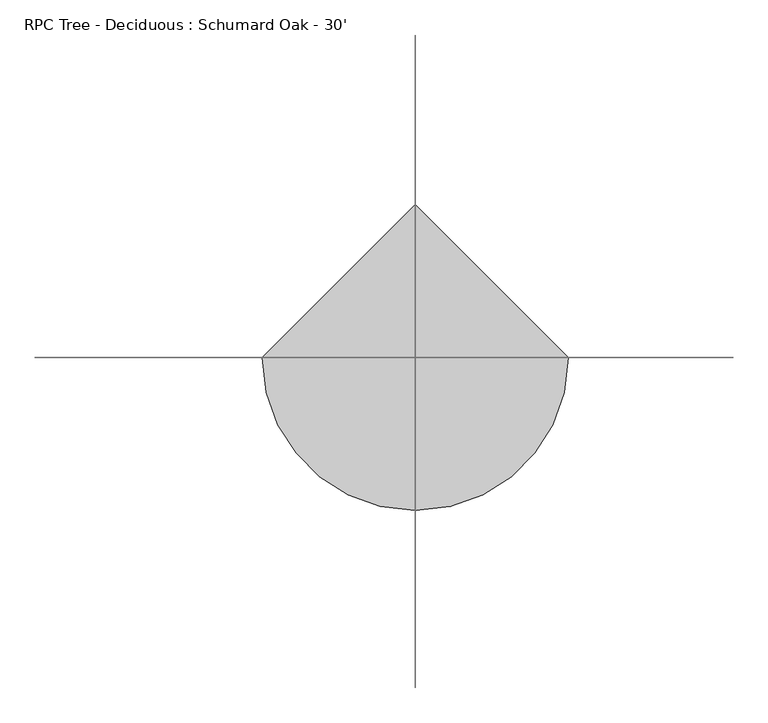
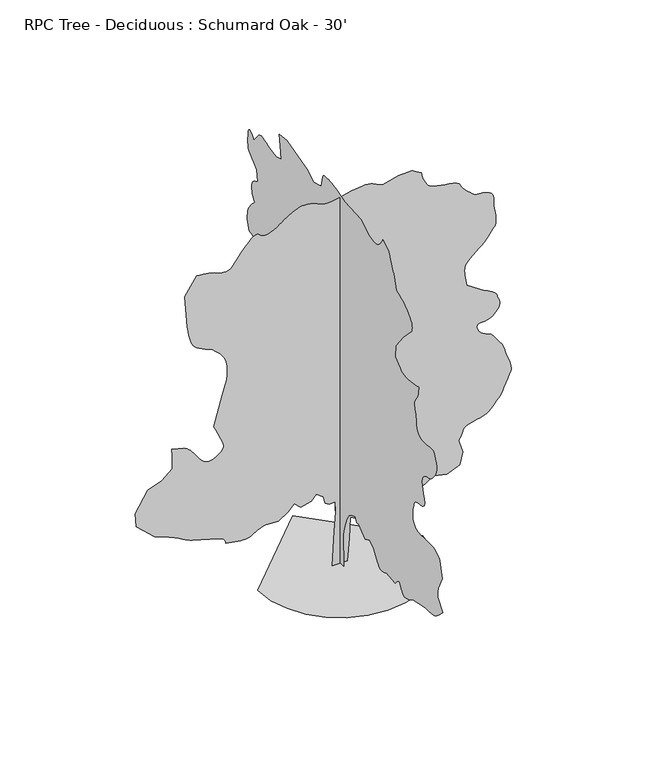
"""IFC4 building model written with IfcOpenShell, lengths in millimetres: geographic element geometry, RPC Tree - Deciduous : Schumard Oak - 30'."""

import ifcopenshell
import ifcopenshell.guid

model = None  # the IFC model being written
_history = None  # IfcOwnerHistory: only IFC2X3 demands one
_inside = {}  # id of a spatial element -> (the spatial element, [elements in it])
_under = {}  # id of a project, library or spatial element -> (it, [spatial elements below it])
_declared = {}  # id of a project -> (the project, [libraries it declares])
_typed = {}  # id of a type object -> (the type object, [elements of that type])
_made_of = {}  # id of a material, layer set ... -> (it, [elements and type objects made of it])


def new_model(schema):
    """Start an empty IFC model of exactly this schema.

    Asked for "IFC4X3", IfcOpenShell would pick the latest addendum, in which some entities
    have other attributes; the version numbers below select the first issue.
    IFC2X3 requires an IfcOwnerHistory on every rooted entity: one is made here for all.
    """
    global model, _history
    if schema == "IFC4X3":
        model = ifcopenshell.file(schema_version=(4, 3, 0, 0))
    else:
        model = ifcopenshell.file(schema=schema)
    _inside.clear()
    _under.clear()
    _declared.clear()
    _typed.clear()
    _made_of.clear()
    _history = None
    if model.schema == "IFC2X3":
        org = make("IfcOrganization", Name="unknown")
        user = make(
            "IfcPersonAndOrganization",
            ThePerson=make("IfcPerson", FamilyName="unknown"),
            TheOrganization=org,
        )
        app = make(
            "IfcApplication",
            ApplicationDeveloper=org,
            Version="unknown",
            ApplicationFullName="unknown",
            ApplicationIdentifier="unknown",
        )
        _history = make(
            "IfcOwnerHistory",
            OwningUser=user,
            OwningApplication=app,
            ChangeAction="ADDED",
            CreationDate=0,
        )
    return model


def make(cls, **values):
    """One entity of the class cls with the attributes given. An attribute that is None is left unset."""
    return model.create_entity(
        cls, **{name: value for name, value in values.items() if value is not None}
    )


def rooted(cls, **values):
    """An entity with a GlobalId (a new one), such as an element, a storey or a relation."""
    return make(cls, GlobalId=ifcopenshell.guid.new(), OwnerHistory=_history, **values)


def si_unit(unit_type, name, prefix=None):
    """IfcSIUnit, for example si_unit("LENGTHUNIT", "METRE", prefix="MILLI")."""
    return make("IfcSIUnit", UnitType=unit_type, Prefix=prefix, Name=name)


def assignment(units):
    """IfcUnitAssignment: the units of a project."""
    return None if units is None else make("IfcUnitAssignment", Units=units)


def point(xyz):
    """IfcCartesianPoint."""
    return None if xyz is None else make("IfcCartesianPoint", Coordinates=xyz)


def direction(xyz):
    """IfcDirection."""
    return None if xyz is None else make("IfcDirection", DirectionRatios=xyz)


def frame(location, z_axis=None, x_axis=None):
    """IfcAxis2Placement3D, a coordinate frame: its origin and axes. An axis left out is left unset."""
    return make(
        "IfcAxis2Placement3D",
        Location=point(location),
        Axis=direction(z_axis),
        RefDirection=direction(x_axis),
    )


def origin():
    """The frame at (0, 0, 0) with its axes left unset."""
    return frame((0.0, 0.0, 0.0))


def place(relative_to, where):
    """IfcLocalPlacement: puts the frame where relative to a parent placement (None: the world)."""
    return make(
        "IfcLocalPlacement", PlacementRelTo=relative_to, RelativePlacement=where
    )


def context(
    kind, dimensions, precision=None, world=None, true_north=None, identifier=None
):
    """IfcGeometricRepresentationContext, for example the 3D "Model" context."""
    return make(
        "IfcGeometricRepresentationContext",
        ContextIdentifier=identifier,
        ContextType=kind,
        CoordinateSpaceDimension=dimensions,
        Precision=precision,
        WorldCoordinateSystem=world,
        TrueNorth=true_north,
    )


def project(units=None, contexts=None):
    """IfcProject with its units and contexts."""
    return rooted(
        "IfcProject",
        Name="project",
        RepresentationContexts=contexts,
        UnitsInContext=assignment(units),
    )


def spatial(cls, under=None, at=None, **own):
    """A site, building, storey or space (cls), placed at a placement, below another one or the project."""
    s = rooted(cls, ObjectPlacement=at, **own)
    if under is not None:
        _under.setdefault(under.id(), (under, []))[1].append(s)
    return s


def point_list(points):
    """IfcCartesianPointList2D or 3D."""
    cls = (
        "IfcCartesianPointList2D" if len(points[0]) == 2 else "IfcCartesianPointList3D"
    )
    return make(cls, CoordList=points)


def triangles(points, corners, closed=None, point_numbers=None):
    """IfcTriangulatedFaceSet: each triangle names its three corners, points numbered from 1."""
    return make(
        "IfcTriangulatedFaceSet",
        Coordinates=point_list(points),
        Closed=closed,
        CoordIndex=corners,
        PnIndex=point_numbers,
    )


def shape(context_of_items, identifier, shape_type, items):
    """IfcShapeRepresentation: the items that make up one representation, for example the "Body"."""
    return make(
        "IfcShapeRepresentation",
        ContextOfItems=context_of_items,
        RepresentationIdentifier=identifier,
        RepresentationType=shape_type,
        Items=items,
    )


def source(mapping_origin, context_of_items, identifier, shape_type, items):
    """IfcRepresentationMap: a shape defined once, which mapped items show again and again."""
    return make(
        "IfcRepresentationMap",
        MappingOrigin=mapping_origin,
        MappedRepresentation=shape(context_of_items, identifier, shape_type, items),
    )


def transform(
    local_origin,
    x_axis=None,
    y_axis=None,
    z_axis=None,
    scale=None,
    scale2=None,
    scale3=None,
    uniform=True,
):
    """IfcCartesianTransformationOperator3D, or its non-uniform kind. x_axis, y_axis, z_axis: its Axis1, 2, 3."""
    if uniform:
        return make(
            "IfcCartesianTransformationOperator3D",
            Axis1=direction(x_axis),
            Axis2=direction(y_axis),
            LocalOrigin=point(local_origin),
            Scale=scale,
            Axis3=direction(z_axis),
        )
    return make(
        "IfcCartesianTransformationOperator3DnonUniform",
        Axis1=direction(x_axis),
        Axis2=direction(y_axis),
        LocalOrigin=point(local_origin),
        Scale=scale,
        Axis3=direction(z_axis),
        Scale2=scale2,
        Scale3=scale3,
    )


def mapped(mapping_source, mapping_target):
    """IfcMappedItem: shows the shape of a source again, moved by a transform."""
    return make(
        "IfcMappedItem", MappingSource=mapping_source, MappingTarget=mapping_target
    )


def made_of(thing, what):
    """Note that an element or type object is made of a material, layer set ...; save() writes the relation."""
    if what is not None:
        _made_of.setdefault(what.id(), (what, []))[1].append(thing)
    return thing


def element(
    cls,
    number,
    at=None,
    inside=None,
    cuts=None,
    type_object=None,
    material=None,
    context=None,
    identifier="Body",
    shape_type=None,
    held_by="IfcProductDefinitionShape",
    body=None,
    shapes=None,
    **own,
):
    """One element of the class cls, such as IfcWall. Its Tag is "e" and its number.

    at: its placement. inside: the storey or other place that contains it. cuts: it is an
    opening in that element (IfcRelVoidsElement). A single representation is given by context,
    identifier, shape_type and body (its items); several are given by shapes. held_by: the class
    of the entity that holds the representations. save() writes the other relations.
    """
    e = rooted(cls, Tag="e%d" % number, ObjectPlacement=at, **own)
    if body is not None:
        shapes = [shape(context, identifier, shape_type, body)]
    if shapes is not None:
        e.Representation = make(held_by, Representations=shapes)
    if inside is not None:
        _inside.setdefault(inside.id(), (inside, []))[1].append(e)
    if cuts is not None:
        rooted(
            "IfcRelVoidsElement", RelatingBuildingElement=cuts, RelatedOpeningElement=e
        )
    if type_object is not None:
        _typed.setdefault(type_object.id(), (type_object, []))[1].append(e)
    return made_of(e, material)


def aggregate(whole, parts):
    """IfcRelAggregates: a whole, such as a stair, and the parts it consists of."""
    return rooted("IfcRelAggregates", RelatingObject=whole, RelatedObjects=parts)


def save(model, path):
    """Write the relations noted so far, then the file.

    IfcRelAggregates (storeys below a building ...), IfcRelContainedInSpatialStructure (elements
    in a storey), IfcRelDefinesByType, IfcRelAssociatesMaterial and IfcRelDeclares: one each for
    every whole, place, type object, material and project.
    """
    for whole, parts in _under.values():
        aggregate(whole, parts)
    for where, things in _inside.values():
        rooted(
            "IfcRelContainedInSpatialStructure",
            RelatedElements=things,
            RelatingStructure=where,
        )
    for kind, things in _typed.values():
        rooted("IfcRelDefinesByType", RelatedObjects=things, RelatingType=kind)
    for what, things in _made_of.values():
        rooted("IfcRelAssociatesMaterial", RelatedObjects=things, RelatingMaterial=what)
    for by, libraries in _declared.values():
        rooted("IfcRelDeclares", RelatingContext=by, RelatedDefinitions=libraries)
    model.write(path)


def rpc_tree_deciduous_schumard_oak_30_cf07c7db(model_context):
    return source(origin(), model_context, "Body", "Tessellation", [
        triangles([(-0.0016958, 164.6246354, 0.0086022), (-0.0016958, -151.6104316, 0.0086022), (-0.0016958, -124.1113561, 783.7227293), (-0.0016958, -179.1089983, 1017.4612965), (-0.0016958, -261.6049622, 1237.4509209), (-0.0016958, -357.8507226, 1388.6927067), (-0.0016958, -467.8454985, 1457.4403999), (-0.0016958, -605.3383779, 1512.436607), (-0.0016958, -660.3370193, 1388.6927067), (-0.0016958, -756.5828161, 1416.1908829), (-0.0016958, -866.5775557, 1306.195998), (-0.0016958, -1017.8194868, 1209.9502739), (-0.0016958, -1196.5619196, 1292.4469826), (-0.0016958, -1361.5527935, 1182.452243), (-0.0016958, -1471.5476784, 989.9607222), (-0.0016958, -1498.1643677, 951.9597713), (-0.0016958, -1525.3829098, 915.7621988), (-0.0016958, -1553.8031227, 883.1739264), (-0.0016958, -1584.0290394, 855.9959341), (-0.0016958, -1616.658007, 836.0340712), (-0.0016958, -1652.2942039, 825.0891724), (-0.0016958, -1691.5371574, 824.9697756), (-0.0016958, -1729.1774471, 831.662681), (-0.0016958, -1760.3255459, 839.8008471), (-0.0016958, -1786.0582775, 849.1404659), (-0.0016958, -1807.4654011, 859.4426714), (-0.0016958, -1825.6238857, 870.4663445), (-0.0016958, -1841.6182583, 881.9725462), (-0.0016958, -1856.5307201, 893.7149254), (-0.0016958, -2214.0131149, 852.4678791), (-0.0016958, -2249.2480282, 893.1561659), (-0.0016958, -2283.7616192, 930.4738735), (-0.0016958, -2316.8324203, 961.0605967), (-0.0016958, -2347.7391094, 981.54314), (-0.0016958, -2375.7578934, 988.5586275), (-0.0016958, -2400.1697754, 978.7389507), (-0.0016958, -2420.2535786, 948.7136032), (-0.0016958, -2440.416156, 905.5412384), (-0.0016958, -2465.389341, 860.9260838), (-0.0016958, -2494.9323051, 818.4750412), (-0.0016958, -2528.8058189, 781.7974108), (-0.0016958, -2566.7735596, 754.4999491), (-0.0016958, -2608.5820541, 740.1896307), (-0.0016958, -2653.9973053, 742.4730669), (-0.0016958, -2699.5395836, 755.8614212), (-0.0016958, -2742.1861084, 772.1352098), (-0.0016958, -2782.4196991, 790.8169184), (-0.0016958, -2820.7484642, 811.421402), (-0.0016958, -2857.6293526, 833.4686754), (-0.0016958, -2893.5448929, 856.475992), (-0.0016958, -2928.9779045, 879.96591), (-0.0016958, -3423.9482735, 976.2117067), (-0.0016958, -3485.6956673, 976.3335743), (-0.0016958, -3546.579451, 977.174366), (-0.0016958, -3605.7868835, 979.4603456), (-0.0016958, -3662.4543549, 983.9078939), (-0.0016958, -3715.7688332, 991.2459635), (-0.0016958, -3764.8925789, 1002.1882462), (-0.0016958, -3808.9361115, 1017.4612965), (-0.0016958, -3851.3797417, 1039.546649), (-0.0016958, -3896.0075409, 1069.5719965), (-0.0016958, -3942.4134293, 1106.2115479), (-0.0016958, -3990.2924835, 1148.1393665), (-0.0016958, -4039.2383331, 1194.0371464), (-0.0016958, -4088.8951859, 1242.5817123), (-0.0016958, -4138.9334106, 1292.4469826), (-0.0016958, -3946.4265564, 1512.436607), (-0.0016958, -3940.7114983, 1553.6455742), (-0.0016958, -3935.9362083, 1594.6132771), (-0.0016958, -3933.0916145, 1635.0983059), (-0.0016958, -3933.1169037, 1674.8646286), (-0.0016958, -3937.0032944, 1713.6657486), (-0.0016958, -3945.7152626, 1751.2679592), (-0.0016958, -3960.1934486, 1787.4247639), (-0.0016958, -4111.425206, 2103.6601124), (-0.0016958, -4015.1842781, 2488.640538), (-0.0016958, -4007.6405525, 2499.2628548), (-0.0016958, -3985.1869812, 2526.4815422), (-0.0016958, -3948.0776184, 2563.3191193), (-0.0016958, -3896.5156494, 2602.8164177), (-0.0016958, -3830.780127, 2637.9697952), (-0.0016958, -3751.1003975, 2661.820665), (-0.0016958, -3657.7046448, 2667.3831161), (-0.0016958, -3553.6406479, 2663.0650658), (-0.0016958, -3446.4524231, 2661.3634254), (-0.0016958, -3343.1000107, 2661.617189), (-0.0016958, -3250.5928665, 2663.0650658), (-0.0016958, -3175.8660324, 2664.970182), (-0.0016958, -3125.9298363, 2666.6718224), (-0.0016958, -3107.7178665, 2667.3831161), (-0.0016958, -3097.049913, 2674.6474983), (-0.0016958, -3069.5669975, 2695.1200859), (-0.0016958, -3031.9495262, 2726.9207611), (-0.0016958, -2990.9793526, 2768.0688309), (-0.0016958, -2953.3874611, 2816.7097572), (-0.0016958, -2925.9045456, 2870.8625565), (-0.0016958, -2915.2365921, 2928.622403), (-0.0016958, -2917.2431557, 2986.3310898), (-0.0016958, -2922.8564758, 3041.9064766), (-0.0016958, -2931.4672874, 3095.6529053), (-0.0016958, -2942.4907425, 3147.977037), (-0.0016958, -2955.3178665, 3199.2087936), (-0.0016958, -2969.3385223, 3249.7039673), (-0.0016958, -2983.9690247, 3299.8436394), (-0.0016958, -2996.0086967, 3314.52472), (-0.0016958, -3009.4706657, 3328.8250099), (-0.0016958, -3025.8280975, 3342.414006), (-0.0016958, -3046.5038704, 3354.9362068), (-0.0016958, -3072.9705688, 3365.9852417), (-0.0016958, -3106.6510712, 3375.2561874), (-0.0016958, -3148.9673836, 3382.3429642), (-0.0016958, -3200.1485619, 3386.6863037), (-0.0016958, -3255.4443146, 3391.740937), (-0.0016958, -3308.7843727, 3403.2725006), (-0.0016958, -3354.1996239, 3427.0722107), (-0.0016958, -3385.6703773, 3468.9315742), (-0.0016958, -3397.1766518, 3534.5906479), (-0.0016958, -3382.6984657, 3629.8406479), (-0.0016958, -3353.0819595, 3737.5114014), (-0.0016958, -3325.8786781, 3836.2667107), (-0.0016958, -3305.152327, 3925.6746254), (-0.0016958, -3294.9921913, 4005.2023293), (-0.0016958, -3299.5387161, 4074.3920013), (-0.0016958, -3322.8306084, 4132.761113), (-0.0016958, -3368.9571533, 4179.8018463), (-0.0016958, -3425.5228867, 4212.7710548), (-0.0016958, -3477.9993347, 4232.964299), (-0.0016958, -3527.3262657, 4246.1975029), (-0.0016958, -3574.5193153, 4258.2118858), (-0.0016958, -3620.493544, 4274.8233719), (-0.0016958, -3666.2390076, 4301.7473099), (-0.0016958, -3712.6954742, 4344.8004959), (-0.0016958, -3760.0411308, 4399.562851), (-0.0016958, -3805.2023277, 4457.9322533), (-0.0016958, -3844.3694138, 4520.1368866), (-0.0016958, -3873.6809967, 4586.4308052), (-0.0016958, -3889.2765564, 4657.068354), (-0.0016958, -3887.295282, 4732.2777168), (-0.0016958, -3863.9272316, 4812.2879494), (-0.0016958, -3835.7077332, 4887.9545517), (-0.0016958, -3816.632444, 4949.7019455), (-0.0016958, -3799.0047409, 4996.9967331), (-0.0016958, -3775.1032928, 5029.3819656), (-0.0016958, -3737.2573471, 5046.3745331), (-0.0016958, -3677.7705711, 5047.4919067), (-0.0016958, -3588.9466324, 5032.2771378), (-0.0016958, -3483.5620766, 5015.437468), (-0.0016958, -3382.266806, 5012.0591858), (-0.0016958, -3289.150106, 5022.1684525), (-0.0016958, -3208.3018433, 5045.7396881), (-0.0016958, -3143.7860138, 5082.7728928), (-0.0016958, -3099.7421906, 5133.2930649), (-0.0016958, -3080.2096619, 5197.2507889), (-0.0016958, -3073.5295464, 5265.5768509), (-0.0016958, -3065.4015541, 5329.5339935), (-0.0016958, -3056.0541595, 5389.9099594), (-0.0016958, -3045.7417076, 5447.3901718), (-0.0016958, -3034.7182526, 5502.7112137), (-0.0016958, -3023.2119781, 5556.5846695), (-0.0016958, -3011.4772293, 5609.7471222), (-0.0016958, -3000.047113, 5648.0755966), (-0.0016958, -2990.8014565, 5686.505809), (-0.0016958, -2985.8485611, 5725.1900757), (-0.0016958, -2987.423465, 5764.2295532), (-0.0016958, -2997.6341789, 5803.7521408), (-0.0016958, -3018.6907425, 5843.8839935), (-0.0016958, -3052.7267464, 5884.7274307), (-0.0016958, -3089.125106, 5934.8418137), (-0.0016958, -3116.6080215, 5997.6815826), (-0.0016958, -3136.4198936, 6065.8297485), (-0.0016958, -3149.7295464, 6131.8187439), (-0.0016958, -3157.7558006, 6188.1815826), (-0.0016958, -3161.6674805, 6227.450116), (-0.0016958, -3162.7089867, 6242.2073547), (-0.0016958, -3142.4395844, 6237.6861191), (-0.0016958, -3088.0074417, 6226.1798447), (-0.0016958, -3009.0387154, 6210.8383392), (-0.0016958, -2915.160434, 6194.7602509), (-0.0016958, -2815.9731743, 6181.0948059), (-0.0016958, -2721.1295448, 6172.9418152), (-0.0016958, -2640.2304131, 6173.4749222), (-0.0016958, -2571.9299309, 6185.3619873), (-0.0016958, -2507.9599983, 6208.094902), (-0.0016958, -2447.5915901, 6239.8452896), (-0.0016958, -2390.1089069, 6278.808609), (-0.0016958, -2334.7901905, 6323.1826447), (-0.0016958, -2280.9167347, 6371.1634369), (-0.0016958, -2227.7621304, 6420.9476074), (-0.0016958, -2241.5111458, 6709.6945175), (-0.0016958, -2543.9897758, 7094.6826462), (-0.0016958, -2887.7283875, 7452.1625702), (-0.0016958, -2893.1132332, 7496.4860275), (-0.0016958, -2895.3482712, 7541.6722229), (-0.0016958, -2891.335144, 7588.5356415), (-0.0016958, -2877.9493332, 7637.9128601), (-0.0016958, -2852.0666107, 7690.6689423), (-0.0016958, -2810.5377502, 7747.6160477), (-0.0016958, -2750.2379425, 7809.6424942), (-0.0016958, -2679.5242355, 7869.2562973), (-0.0016958, -2608.8108192, 7919.4724182), (-0.0016958, -2538.10467, 7961.8901779), (-0.0016958, -2467.3935791, 7998.0344833), (-0.0016958, -2396.6824883, 8029.5052368), (-0.0016958, -2325.9712521, 8057.8517624), (-0.0016958, -2255.2601612, 8084.6233841), (-0.0016958, -2234.6175259, 8155.1336151), (-0.0016958, -2213.8530956, 8224.4503143), (-0.0016958, -2192.8472557, 8291.3537888), (-0.0016958, -2171.4808273, 8354.651088), (-0.0016958, -2149.6341957, 8413.1219376), (-0.0016958, -2127.1881821, 8465.5983856), (-0.0016958, -2104.0183754, 8510.8607391), (-0.0016958, -2078.3235775, 8560.2129593), (-0.0016958, -2049.9822842, 8621.0970337), (-0.0016958, -2021.4021973, 8686.5529221), (-0.0016958, -1994.9862225, 8749.5955856), (-0.0016958, -1973.1395908, 8803.2917267), (-0.0016958, -1958.2679695, 8840.6039841), (-0.0016958, -1952.7738281, 8854.5996414), (-0.0016958, -1719.0353336, 8992.089505), (-0.0016958, -1707.0516174, 8968.3915329), (-0.0016958, -1693.863905, 8943.9819763), (-0.0016958, -1678.2681999, 8918.1248337), (-0.0016958, -1659.0683544, 8890.1085205), (-0.0016958, -1635.057756, 8859.1970352), (-0.0016958, -1605.0324085, 8824.678212), (-0.0016958, -1567.7934025, 8785.841629), (-0.0016958, -1522.9369835, 8752.2122864), (-0.0016958, -1471.5882282, 8732.2983856), (-0.0016958, -1414.8268673, 8723.7896027), (-0.0016958, -1353.7372822, 8724.4244476), (-0.0016958, -1289.3990582, 8731.9175949), (-0.0016958, -1222.896722, 8743.9825562), (-0.0016958, -1155.3123299, 8758.3334244), (-0.0016958, -852.8259968, 8964.5813004), (-0.0016958, -192.8582863, 9005.8311081), (-0.0016958, -107.5965211, 9029.2756073), (-0.0016958, -23.416737, 9052.008522), (-0.0016958, 58.5983536, 9073.2938507), (-0.0016958, 137.366361, 9092.4200089), (-0.0016958, 211.8051857, 9108.6504135), (-0.0016958, 280.8327856, 9121.2740616), (-0.0016958, 343.3650879, 9129.57995), (-0.0016958, 405.0185557, 9135.9045639), (-0.0016958, 469.5549508, 9141.5181747), (-0.0016958, 533.1311937, 9144.0075577), (-0.0016958, 591.8966838, 9140.9594879), (-0.0016958, 642.0033274, 9129.9863205), (-0.0016958, 679.6029219, 9108.6504135), (-0.0016958, 700.8500261, 9074.5891205), (-0.0016958, 769.5952486, 8799.5832321), (-0.0016958, 1072.081509, 8717.1091965), (-0.0016958, 1347.0698112, 8882.0822662), (-0.0016958, 1690.8031906, 8964.5813004), (-0.0016958, 2144.5313095, 9102.0717453), (-0.0016958, 2447.0174973, 9060.8225189), (-0.0016958, 2419.5169956, 8799.5832321), (-0.0016958, 2364.5209339, 8497.1197174), (-0.0016958, 2584.5030006, 8428.361705), (-0.0016958, 2804.4924797, 8469.6115128), (-0.0016958, 2889.5570549, 8501.5647949), (-0.0016958, 2972.3357231, 8530.7490601), (-0.0016958, 3050.5425774, 8554.3964539), (-0.0016958, 3121.8911293, 8569.7385406), (-0.0016958, 3184.1210518, 8574.0307205), (-0.0016958, 3234.8958595, 8564.480722), (-0.0016958, 3271.9799332, 8538.3439453), (-0.0016958, 3478.2280998, 8290.8712601), (-0.0016958, 3525.090937, 8345.6591949), (-0.0016958, 3570.2521339, 8393.3603531), (-0.0016958, 3612.0606285, 8426.8885391), (-0.0016958, 3648.8144897, 8439.1058167), (-0.0016958, 3678.8373665, 8422.9515701), (-0.0016958, 3700.4526169, 8371.313443), (-0.0016958, 3711.9588913, 8277.1046585), (-0.0016958, 3715.4389114, 8172.4819748), (-0.0016958, 3714.6005905, 8091.684581), (-0.0016958, 3710.155513, 8030.6987686), (-0.0016958, 3702.8149727, 7985.6137299), (-0.0016958, 3693.3152618, 7952.4163376), (-0.0016958, 3682.3679649, 7927.1684601), (-0.0016958, 3670.7093742, 7905.8831314), (-0.0016958, 3354.4789673, 7644.6438446), (-0.0016958, 3326.9707626, 7355.921933), (-0.0016958, 3370.9384277, 7337.989888), (-0.0016958, 3413.6102417, 7318.6346741), (-0.0016958, 3453.615358, 7296.384288), (-0.0016958, 3489.6326363, 7269.8161423), (-0.0016958, 3520.3920959, 7237.4564896), (-0.0016958, 3544.5220184, 7197.8833237), (-0.0016958, 3560.7018448, 7149.674057), (-0.0016958, 3566.8994316, 7096.6389221), (-0.0016958, 3562.9624626, 7043.6032059), (-0.0016958, 3550.618158, 6990.568071), (-0.0016958, 3531.5425781, 6937.5329361), (-0.0016958, 3507.4126556, 6884.4978012), (-0.0016958, 3479.904451, 6831.4626663), (-0.0016958, 3450.7198952, 6778.4269501), (-0.0016958, 3494.7381386, 6734.2313919), (-0.0016958, 3537.6640068, 6689.8829361), (-0.0016958, 3578.4309952, 6645.3060059), (-0.0016958, 3615.9470192, 6600.3732834), (-0.0016958, 3649.1447021, 6554.9580322), (-0.0016958, 3676.9322502, 6508.9329346), (-0.0016958, 3698.2175789, 6462.1968338), (-0.0016958, 3713.4829262, 6416.6548462), (-0.0016958, 3724.4305138, 6374.0080307), (-0.0016958, 3731.7710541, 6333.77444), (-0.0016958, 3736.2161316, 6295.4459656), (-0.0016958, 3738.5020386, 6258.5650772), (-0.0016958, 3739.3400688, 6222.6492462), (-0.0016958, 3739.4670959, 6187.2165253), (-0.0016958, 3656.9680618, 5953.4854431), (-0.0016958, 3618.6901657, 5947.3387253), (-0.0016958, 3580.5140076, 5939.7694199), (-0.0016958, 3542.591613, 5929.304361), (-0.0016958, 3505.0250107, 5914.5215424), (-0.0016958, 3467.9665169, 5893.9477982), (-0.0016958, 3431.4664192, 5866.1599594), (-0.0016958, 3395.728775, 5829.7366013), (-0.0016958, 3363.165937, 5786.4799393), (-0.0016958, 3335.6830215, 5739.6171021), (-0.0016958, 3312.3911293, 5689.7567734), (-0.0016958, 3292.4522301, 5637.4838013), (-0.0016958, 3275.0532921, 5583.4068695), (-0.0016958, 3259.3559944, 5528.1364059), (-0.0016958, 3244.4717285, 5472.2566772), (-0.0016958, 3212.2896812, 5428.0349579), (-0.0016958, 3181.4287743, 5383.7120819), (-0.0016958, 3153.2092758, 5339.1351517), (-0.0016958, 3128.9523262, 5294.1768494), (-0.0016958, 3110.0037735, 5248.7615982), (-0.0016958, 3097.6341797, 5202.7620804), (-0.0016958, 3093.2399712, 5156.026561), (-0.0016958, 3106.9812836, 4784.7797447), (-0.0016958, 3139.1630402, 4781.5284897), (-0.0016958, 3170.049527, 4776.4738564), (-0.0016958, 3198.2690254, 4767.8377556), (-0.0016958, 3222.5006859, 4753.7662308), (-0.0016958, 3241.4745277, 4732.4809021), (-0.0016958, 3253.8188324, 4702.1533928), (-0.0016958, 3258.2383301, 4661.0306122), (-0.0016958, 3257.0192184, 4613.5073502), (-0.0016958, 3253.6665161, 4565.2219254), (-0.0016958, 3248.4848557, 4516.377523), (-0.0016958, 3241.8808983, 4467.0253029), (-0.0016958, 3234.1845657, 4417.3175812), (-0.0016958, 3225.7516502, 4367.3810944), (-0.0016958, 3216.988813, 4317.2922913), (-0.0016958, 3203.2219208, 4042.311692), (-0.0016958, 3464.4612076, 4056.0785843), (-0.0016958, 3753.208699, 4111.0694138), (-0.0016958, 3814.6511696, 4090.2669044), (-0.0016958, 3873.5792587, 4068.37202), (-0.0016958, 3927.4527145, 4044.3182556), (-0.0016958, 3973.7568649, 4017.0132362), (-0.0016958, 4009.9520393, 3985.3901665), (-0.0016958, 4033.523275, 3948.3569618), (-0.0016958, 4041.9306107, 3904.8212471), (-0.0016958, 4039.5429657, 3849.6778107), (-0.0016958, 4032.8119812, 3780.081768), (-0.0016958, 4022.448951, 3698.4716331), (-0.0016958, 4009.2407455, 3607.2347603), (-0.0016958, 3993.8483711, 3508.7840836), (-0.0016958, 3977.00812, 3405.5078293), (-0.0016958, 3959.4568657, 3299.8436394), (-0.0016958, 3835.7077332, 2969.87192), (-0.0016958, 3768.1185448, 2931.9498161), (-0.0016958, 3701.6211502, 2896.3136192), (-0.0016958, 3637.2829262, 2865.2492363), (-0.0016958, 3576.1959572, 2841.0431557), (-0.0016958, 3519.4267479, 2825.9554138), (-0.0016958, 3468.0679642, 2822.3233681), (-0.0016958, 3423.2113998, 2832.3817657), (-0.0016958, 3038.248851, 2997.3548355), (-0.0016958, 2653.2607224, 2873.6312828), (-0.0016958, 2378.2699493, 2681.1244286), (-0.0016958, 2103.2842632, 2268.651059), (-0.0016958, 2076.6675739, 2227.6428062), (-0.0016958, 2049.4488865, 2188.0796688), (-0.0016958, 2021.0263481, 2151.4021111), (-0.0016958, 1990.8027569, 2119.0526321), (-0.0016958, 1958.1739346, 2092.4764927), (-0.0016958, 1922.5377377, 2073.1141571), (-0.0016958, 1883.2946388, 2062.4105953), (-0.0016958, 1844.1303143, 2058.8443886), (-0.0016958, 1807.3715115, 2059.123732), (-0.0016958, 1770.371299, 2062.0498615), (-0.0016958, 1730.4881229, 2066.4186356), (-0.0016958, 1685.070401, 2071.0288193), (-0.0016958, 1631.4762886, 2074.6762711), (-0.0016958, 1567.0592903, 2076.1596107), (-0.0016958, 1497.9510086, 2070.950045), (-0.0016958, 1431.730632, 2056.3577671), (-0.0016958, 1367.9130157, 2033.9498325), (-0.0016958, 1306.020718, 2005.2883553), (-0.0016958, 1245.5712101, 1971.9382107), (-0.0016958, 1186.0844341, 1935.4612221), (-0.0016958, 1127.0801868, 1897.4196487), (-0.0016958, 1044.5834782, 1663.6810089), (-0.0016958, 810.8448383, 1402.4418674), (-0.0016958, 778.5741337, 1367.4862976), (-0.0016958, 741.256426, 1333.2546661), (-0.0016958, 699.7273476, 1299.622562), (-0.0016958, 654.8303061, 1266.4729866), (-0.0016958, 607.408455, 1233.6815289), (-0.0016958, 558.3051295, 1201.1339516), (-0.0016958, 508.3585416, 1168.7032276), (-0.0016958, 425.8618329, 1457.4403999), (-0.0016958, 288.3689717, 1649.9293774), (-0.0016958, 233.3715837, 1526.1856224), (-0.0016958, 192.1232112, 1333.696645), (-0.0016958, 178.3741776, 989.9607222), (-0.0016958, 150.8753565, 508.7344634), (170.3625119, 0.000436, 0.0217742), (-187.1199193, 0.000436, 0.0217742), (-132.1230309, 0.000387, 824.9824928), (-104.6242098, 0.0003581, 1306.2087879), (-118.3734886, 0.0003434, 1553.698914), (-255.8671038, 0.0003442, 1539.9498985), (-352.1128461, 0.000341, 1594.9459602), (-393.359965, 0.0003302, 1773.6885384), (-558.3534187, 0.0003237, 1883.6832779), (-668.3482309, 0.000331, 1759.9395229), (-915.8358135, 0.0003352, 1691.1918297), (-1067.0802881, 0.0003271, 1828.6846001), (-1218.3221466, 0.000336, 1677.4428143), (-1438.311771, 0.0003442, 1539.9498985), (-1768.2961349, 0.0003434, 1553.698914), (-1933.2869362, 0.0003476, 1484.9512207), (-1968.7250347, 0.0003491, 1458.6138748), (-2004.6407204, 0.0003507, 1433.3612011), (-2041.5189926, 0.000352, 1410.2726395), (-2079.8425255, 0.0003531, 1390.4301006), (-2120.0889061, 0.0003541, 1374.915786), (-2162.738047, 0.0003547, 1364.8142223), (-2208.2752384, 0.0003549, 1361.2074657), (-2259.0244663, 0.0003549, 1362.8101295), (-2316.2658852, 0.0003547, 1367.3008438), (-2378.9175842, 0.0003541, 1374.1944637), (-2445.902449, 0.0003536, 1383.0132568), (-2516.1310112, 0.0003531, 1393.2749851), (-2588.5161278, 0.0003523, 1404.4991547), (-2661.9982704, 0.0003518, 1416.2061436), (-2665.4018417, 0.0003499, 1445.5887978), (-2671.5741394, 0.0003481, 1474.4889233), (-2683.2835991, 0.0003465, 1502.428933), (-2703.2986565, 0.0003449, 1528.9262981), (-2734.3630394, 0.0003434, 1553.4981995), (-2779.2448929, 0.0003421, 1575.6648697), (-2840.7382324, 0.000341, 1594.9459602), (-3445.7158401, 0.0003302, 1773.6885384), (-3495.0936401, 0.0003295, 1789.3602562), (-3547.8494316, 0.0003281, 1811.5293972), (-3602.2815742, 0.0003266, 1838.265556), (-3656.7140076, 0.0003247, 1867.6482101), (-3709.469799, 0.0003229, 1897.7523319), (-3758.8728882, 0.0003213, 1926.6550735), (-3803.1957642, 0.0003197, 1952.4285004), (-3850.8716331, 0.0003182, 1977.2011162), (-3910.0790657, 0.0003166, 2004.1403149), (-3978.8876564, 0.0003148, 2032.8804211), (-4055.4181595, 0.0003132, 2063.0657879), (-4137.7140083, 0.0003113, 2094.3332108), (-4223.8456696, 0.0003092, 2126.3194851), (-4311.9327347, 0.0003074, 2158.668964), (-4738.1450912, 0.0002835, 2557.4011665), (-4765.6532959, 0.0002638, 2887.3725952), (-4476.9060951, 0.000236, 3354.8600487), (-4146.9343758, 0.0002287, 3478.6088905), (-3899.4364014, 0.0002163, 3684.8570572), (-3899.4364014, 0.0001977, 4001.0874641), (-3913.2032936, 0.0001877, 4166.0858231), (-3624.4558022, 0.0001919, 4097.3281013), (-3591.9438332, 0.0001932, 4076.3729851), (-3558.8475975, 0.0001945, 4053.3607269), (-3524.5322502, 0.0001961, 4026.2588928), (-3488.4135246, 0.0001979, 3993.03563), (-3449.8815742, 0.0002006, 3951.6082169), (-3408.3524231, 0.0002037, 3899.9953789), (-3363.216806, 0.0002074, 3836.0888145), (-3317.4713425, 0.0002113, 3768.956575), (-3273.4275192, 0.000215, 3709.7491425), (-3229.3839867, 0.0002179, 3659.6856285), (-3183.6385231, 0.0002203, 3619.9601463), (-3134.5403572, 0.0002221, 3591.765937), (-3080.387558, 0.0002229, 3576.3482735), (-3019.4781944, 0.0002229, 3574.8495277), (-2952.9046417, 0.0002221, 3590.0895859), (-2885.848851, 0.0002203, 3620.9507835), (-2822.8567657, 0.0002176, 3662.8860146), (-2768.5513596, 0.0002147, 3711.2984665), (-2727.4541588, 0.0002119, 3761.6413239), (-2704.1622665, 0.000209, 3809.3427727), (-2703.2480782, 0.0002066, 3849.8304176), (-2719.4531937, 0.000204, 3893.6198959), (-2743.5831161, 0.0002006, 3952.5479851), (-2774.3172867, 0.0001961, 4024.0997223), (-2810.3598541, 0.0001914, 4105.735437), (-2850.3649704, 0.0001861, 4194.9657463), (-2893.0114952, 0.0001803, 4289.2506889), (-2936.9788696, 0.0001746, 4386.0755928), (-2744.4975952, 0.0001328, 5087.2685486), (-2718.1576332, 0.0001281, 5166.6433548), (-2692.9100464, 0.0001234, 5244.9263672), (-2669.8216301, 0.0001189, 5321.050209), (-2649.9841782, 0.0001145, 5393.948085), (-2634.4647766, 0.0001105, 5462.477623), (-2624.3555099, 0.0001066, 5525.6220245), (-2620.7487534, 0.0001034, 5582.263916), (-2621.6885216, 0.0001, 5637.5343796), (-2624.7618805, 9.66e-05, 5696.1831253), (-2630.5022278, 9.29e-05, 5756.5079315), (-2639.366803, 8.93e-05, 5816.8333191), (-2651.8128456, 8.58e-05, 5875.4820648), (-2668.3737534, 8.24e-05, 5930.7525284), (-2689.5064751, 7.95e-05, 5980.9936478), (-2716.6844673, 7.67e-05, 6027.7297485), (-2750.3649696, 7.4e-05, 6073.7542648), (-2789.4303177, 7.14e-05, 6119.169516), (-2832.8390053, 6.85e-05, 6164.1022385), (-2879.4986572, 6.59e-05, 6208.6791687), (-2928.3430595, 6.33e-05, 6253.002626), (-2978.2286774, 6.06e-05, 6297.223764), (-3057.4511673, 5.88e-05, 6329.6851547), (-3134.6165154, 5.67e-05, 6362.5273361), (-3207.6922874, 5.49e-05, 6396.0805206), (-3274.6213417, 5.28e-05, 6430.7010818), (-3333.3971146, 5.07e-05, 6466.7942276), (-3381.9365936, 4.83e-05, 6504.6657532), (-3418.2076355, 4.59e-05, 6544.7214478), (-3446.7573463, 4.28e-05, 6598.1123749), (-3473.1478867, 3.86e-05, 6670.5027237), (-3496.8717293, 3.36e-05, 6753.9668152), (-3517.4710533, 2.84e-05, 6840.5557159), (-3534.4636208, 2.34e-05, 6922.3181671), (-3547.3669029, 1.94e-05, 6991.3558136), (-3555.7233696, 1.65e-05, 7039.6918167), (-3610.7144897, -2.94e-05, 7809.6424942), (-3335.7086014, -5.49e-05, 8235.8804306), (-3262.2517479, -5.43e-05, 8226.9396973), (-3189.8616898, -5.38e-05, 8217.4146973), (-3119.6305115, -5.3e-05, 8206.6705856), (-3052.6252991, -5.22e-05, 8194.1225143), (-2989.9887154, -5.15e-05, 8179.162381), (-2932.7372681, -5.04e-05, 8161.2041748), (-2881.9880402, -4.91e-05, 8139.6397934), (-2830.4004913, -4.78e-05, 8118.7864151), (-2772.3107231, -4.7e-05, 8104.2064911), (-2711.3504906, -4.65e-05, 8097.069136), (-2651.1018425, -4.67e-05, 8098.5934616), (-2595.1709541, -4.73e-05, 8109.9724182), (-2547.1901619, -4.86e-05, 8132.4262802), (-2510.7589554, -5.07e-05, 8167.1224182), (-2290.7694763, -6.8e-05, 8455.8699097), (-2232.0038773, -7.19e-05, 8523.1291763), (-2174.2011555, -7.59e-05, 8587.3915329), (-2118.3236069, -7.93e-05, 8645.6333267), (-2065.3290218, -8.22e-05, 8694.8588104), (-2016.1850739, -8.45e-05, 8732.0699112), (-1971.8492626, -8.58e-05, 8754.2185593), (-1933.2869362, -8.61e-05, 8758.3590042), (-1902.260923, -8.53e-05, 8748.0212631), (-1877.0081039, -8.43e-05, 8731.181012), (-1853.1982201, -8.32e-05, 8711.4450073), (-1826.5002857, -8.22e-05, 8692.4455856), (-1792.5886929, -8.11e-05, 8677.7900848), (-1747.1302757, -8.09e-05, 8671.0591003), (-1685.7992809, -8.11e-05, 8675.8593887), (-1612.5227943, -8.24e-05, 8696.712767), (-1537.32346, -8.43e-05, 8731.5112244), (-1465.0070892, -8.69e-05, 8773.9795624), (-1400.3895218, -8.95e-05, 8817.9216476), (-1348.2787491, -9.19e-05, 8857.0378647), (-1313.4833439, -9.35e-05, 8885.1047562), (-1300.8163845, -9.42e-05, 8895.8488678), (-1285.3045406, -9.48e-05, 8905.7802383), (-1244.0574944, -9.63e-05, 8931.6123825), (-1185.0100084, -9.84e-05, 8967.2741592), (-1116.1022959, -0.0001008, 9006.7961655), (-1045.2718082, -0.0001029, 9044.1595825), (-980.4534536, -0.0001047, 9073.344429), (-929.5848289, -0.0001055, 9088.3307236), (-881.3222952, -0.0001058, 9091.6578461), (-821.2740709, -0.0001058, 9089.7021515), (-752.8083372, -0.0001053, 9082.2090042), (-679.2905136, -0.0001045, 9068.9505112), (-604.0912156, -0.0001034, 9049.6714554), (-530.573392, -0.0001019, 9024.1189453), (-462.1076583, -0.0001, 8992.089505), (-389.2730779, -9.84e-05, 8965.9533096), (-302.0062388, -9.79e-05, 8956.4283096), (-202.713753, -9.79e-05, 8960.7204895), (-93.8012603, -9.9e-05, 8976.0625763), (22.3266441, -0.0001003, 8999.7099701), (143.2647473, -0.0001021, 9028.8942352), (266.608781, -0.000104, 9060.8475174), (351.7496415, -0.0001047, 9072.3793716), (435.0871056, -0.0001053, 9082.4886383), (514.8177767, -0.0001058, 9089.7021515), (589.1356968, -0.0001058, 9092.597905), (656.2400311, -0.0001058, 9089.7021515), (714.324785, -0.000105, 9079.5928848), (761.584037, -0.000104, 9060.8475174), (801.2284195, -0.0001026, 9038.8767654), (837.987295, -0.0001016, 9019.8011856), (872.3408667, -0.0001005, 9003.1132507), (904.7690472, -9.98e-05, 8988.356012), (935.7570539, -9.9e-05, 8975.0719391), (965.779858, -9.82e-05, 8962.7017639), (995.3226768, -9.74e-05, 8950.8402786), (1352.8050716, -0.0001032, 9047.0809158), (1669.0404202, -0.000104, 9060.8475174), (1889.0325153, -9.66e-05, 8937.0986755), (1892.1974384, -9.48e-05, 8904.5611267), (1896.6881527, -9.27e-05, 8871.1602585), (1903.8228916, -9.06e-05, 8836.0827484), (1914.9278824, -8.85e-05, 8798.4908569), (1931.3210678, -8.58e-05, 8757.5206833), (1954.3308552, -8.32e-05, 8712.3339066), (1985.2757687, -8.03e-05, 8662.118367), (2016.3831722, -7.74e-05, 8616.1438477), (2042.1971489, -7.56e-05, 8582.1842926), (2067.531213, -7.4e-05, 8557.1398911), (2097.1958267, -7.27e-05, 8537.8358368), (2135.9969467, -7.19e-05, 8521.1990616), (2188.7502674, -7.09e-05, 8504.1047562), (2260.2639256, -6.96e-05, 8483.3781143), (2348.4121788, -6.85e-05, 8463.4136353), (2443.5351517, -6.75e-05, 8448.2500259), (2539.1383278, -6.67e-05, 8434.3055283), (2628.7244293, -6.56e-05, 8417.9478058), (2705.8133286, -6.43e-05, 8395.5701019), (2763.9030968, -6.25e-05, 8363.5918213), (2796.4915146, -5.99e-05, 8318.3794647), (2820.5705681, -5.67e-05, 8265.7507004), (2856.206765, -5.36e-05, 8213.8329391), (2901.4696999, -5.04e-05, 8162.5250244), (2954.4286766, -4.75e-05, 8111.6996384), (3013.1535805, -4.44e-05, 8061.2300446), (3075.7137154, -4.15e-05, 8011.0139236), (3140.2298355, -3.83e-05, 7960.8995407), (3230.9333107, -3.78e-05, 7951.6035965), (3317.928582, -3.73e-05, 7939.5386353), (3397.4559952, -3.62e-05, 7921.9362213), (3465.8073463, -3.47e-05, 7896.027919), (3519.2235626, -3.23e-05, 7859.0708725), (3554.0217293, -2.94e-05, 7808.2966461), (3566.4421921, -2.55e-05, 7740.9100616), (3567.2549332, -2.13e-05, 7670.7044632), (3569.4902618, -1.76e-05, 7612.0812973), (3572.9447021, -1.47e-05, 7563.0337097), (3577.3641998, -1.23e-05, 7521.7077438), (3582.4949913, -1.02e-05, 7486.1732849), (3588.1086021, -8.1e-06, 7454.4484772), (3593.9503967, -6.6e-06, 7424.6799454), (3605.4566711, -2.4e-06, 7354.1947128), (3615.2865944, 1.8e-06, 7285.1832275), (3621.7382355, 5.8e-06, 7219.0413345), (3623.1352432, 9.5e-06, 7157.2177826), (3617.8009758, 1.29e-05, 7101.1851563), (3604.0596634, 1.58e-05, 7052.3666245), (3580.2090843, 1.81e-05, 7012.1836121), (3549.779837, 2.05e-05, 6973.6772415), (3516.9376556, 2.31e-05, 6929.6084198), (3480.9965355, 2.6e-05, 6881.221257), (3441.1948952, 2.89e-05, 6829.7098663), (3396.8208595, 3.2e-05, 6776.2933594), (3347.138427, 3.54e-05, 6722.1408508), (3291.4615929, 3.86e-05, 6668.4452911), (3226.8184456, 4.2e-05, 6613.0986694), (3154.6824417, 4.54e-05, 6553.8912369), (3081.1241409, 4.91e-05, 6492.0421051), (3012.1376541, 5.28e-05, 6428.7453873), (2953.7429626, 5.67e-05, 6365.2196136), (2911.9344681, 6.04e-05, 6302.6338989), (2892.7321518, 6.41e-05, 6242.2329346), (2889.6587929, 6.75e-05, 6182.4918137), (2891.6144875, 7.11e-05, 6121.3286865), (2897.7867851, 7.48e-05, 6058.9464478), (2907.3370743, 7.88e-05, 5995.6241501), (2919.4020355, 8.24e-05, 5931.5652695), (2933.1436386, 8.64e-05, 5867.0238602), (2947.7232719, 9.03e-05, 5802.2533951), (3360.2196053, 0.0001066, 5527.2475067), (3376.1959557, 0.0001071, 5520.1357315), (3417.4457634, 0.0001082, 5500.475885), (3473.8591805, 0.00011, 5470.9864059), (3535.3019417, 0.0001121, 5434.2584152), (3591.7153587, 0.0001147, 5392.9830276), (3632.9648758, 0.0001171, 5349.7525269), (3648.9415169, 0.0001197, 5307.2580276), (3657.5267487, 0.0001221, 5267.1511734), (3677.1610153, 0.0001244, 5227.0193207), (3698.7256874, 0.0001271, 5183.5347656), (3713.0765556, 0.0001302, 5133.2930649), (3711.0699921, 0.0001336, 5072.9682587), (3683.5870766, 0.0001381, 4999.1814835), (3621.4586014, 0.0001436, 4908.5282959), (3535.7588905, 0.0001481, 4831.4141075), (3447.6462456, 0.0001504, 4791.5613075), (3363.1403572, 0.0001515, 4775.7881424), (3288.2612068, 0.0001517, 4770.8096672), (3229.0029053, 0.0001523, 4763.4182579), (3191.4110138, 0.0001536, 4740.4312889), (3181.4796432, 0.0001567, 4688.5388168), (3195.7796425, 0.0001604, 4623.8450912), (3225.2438324, 0.0001635, 4569.9716354), (3267.3316704, 0.0001664, 4525.1153618), (3319.528775, 0.0001685, 4487.4723106), (3379.2948944, 0.0001704, 4455.2396851), (3444.1156471, 0.0001722, 4426.6393959), (3511.4510719, 0.0001738, 4399.8169052), (3578.7612076, 0.0001788, 4314.6761719), (3643.3026169, 0.0001838, 4231.3385262), (3702.3068642, 0.0001885, 4151.6079277), (3753.0055138, 0.000193, 4077.2874641), (3792.6548378, 0.0001972, 4010.1805138), (3818.4611115, 0.0002006, 3952.0907455), (3827.6814789, 0.0002032, 3904.8468269), (3838.9084099, 0.0002066, 3848.3063828), (3866.9753014, 0.0002116, 3767.5086983), (3903.4498192, 0.0002171, 3671.7761696), (3939.9240463, 0.0002231, 3570.531768), (3967.9912285, 0.0002289, 3473.1225975), (3979.2178688, 0.0002342, 3388.9469215), (3965.1716331, 0.0002378, 3327.351844), (3932.583506, 0.0002413, 3266.5442184), (3894.7119804, 0.0002462, 3184.3498169), (3852.9799347, 0.000252, 3089.6076347), (3808.8599533, 0.0002578, 2991.2842758), (3763.7496254, 0.0002633, 2898.2440247), (3719.1471153, 0.000268, 2819.4023254), (3676.4497215, 0.0002714, 2763.6493332), (3635.0475975, 0.0002741, 2719.4784828), (3592.6804161, 0.000277, 2671.193058), (3548.3828293, 0.0002798, 2621.4853363), (3501.189489, 0.0002827, 2572.9967262), (3450.1609177, 0.0002854, 2528.3384056), (3394.3317673, 0.0002877, 2490.1773628), (3332.7114006, 0.0002893, 2461.1552971), (3259.8893921, 0.0002906, 2439.6287041), (3175.9677704, 0.0002919, 2420.2688393), (3088.4646812, 0.000293, 2400.1850361), (3004.822403, 0.0002943, 2376.4944763), (2932.457634, 0.0002961, 2346.3115803), (2878.8638123, 0.0002985, 2306.7459721), (2851.4823441, 0.0003016, 2254.9146881), (2836.8265526, 0.0003048, 2202.96408), (2818.2846611, 0.0003071, 2162.5576801), (2798.8027107, 0.000309, 2130.0888771), (2781.2514565, 0.0003108, 2101.9481529), (2768.5004906, 0.0003124, 2074.5288963), (2763.4461479, 0.0003142, 2044.2240601), (2768.9833099, 0.0003163, 2007.4271782), (2851.4823441, 0.0003321, 1746.1905075), (2782.7499115, 0.0003499, 1443.7041744), (2480.25355, 0.0003573, 1319.9602741), (2177.7672169, 0.0003533, 1388.7054966), (1875.2810291, 0.0003646, 1196.2165192), (1655.2914047, 0.0003573, 1319.9602741), (1339.0560562, 0.0003491, 1457.4531898), (1318.3321758, 0.0003499, 1445.3856125), (1297.0062973, 0.0003507, 1431.6365971), (1274.4790386, 0.0003518, 1414.5220894), (1250.1457855, 0.0003531, 1392.3529484), (1223.4097721, 0.0003547, 1363.4528229), (1193.6663115, 0.000357, 1326.1325718), (1160.3160942, 0.0003599, 1278.7106117), (1125.360597, 0.0003628, 1228.8834206), (1091.1289656, 0.0003654, 1184.8296415), (1057.4968615, 0.0003678, 1145.5866154), (1024.3447426, 0.0003699, 1110.1916828), (991.5558283, 0.0003717, 1077.6822573), (959.0057076, 0.0003736, 1047.0980776), (926.577527, 0.0003754, 1017.4740137), (967.8245733, 0.0003927, 728.7367687), (944.1340136, 0.0003933, 720.0372271), (919.7220589, 0.0003935, 712.1810205), (893.867387, 0.000394, 706.0087955), (865.8460596, 0.0003943, 702.3613438), (834.9418413, 0.0003943, 702.0819277), (800.428323, 0.000394, 706.0087955), (761.584037, 0.0003935, 714.9876806), (721.1370872, 0.0003925, 729.9787714), (682.1353254, 0.0003914, 750.743347), (644.3350164, 0.0003898, 776.3186028), (607.4948233, 0.000388, 805.7419521), (571.3785321, 0.0003862, 838.0508085), (535.7422989, 0.0003841, 872.28244), (500.3473663, 0.000382, 907.4792015), (239.1089334, 0.0003738, 1044.9720446), (211.6111206, 0.000404, 536.2452115), (-1916.7566952, 0.0, 0.0), (-1866.0836254, -439.194304, 0.0), (-1721.7683064, -842.5237186, 0.0), (-1495.3652653, -1198.4313549, 0.0), (-1198.4313549, -1495.3652653, 0.0), (-842.5237186, -1721.7683064, 0.0), (-439.194304, -1866.0836254, 0.0), (8.38e-05, -1916.7566952, 0.0), (439.194304, -1866.0836254, 0.0), (842.5237186, -1721.7683064, 0.0), (1198.4313549, -1495.3652653, 0.0), (1495.3652653, -1198.4313549, 0.0), (1721.7683064, -842.5237186, 0.0), (1866.0836254, -439.194304, 0.0), (1916.7566952, 0.0001675, 0.0), (-0.0002514, 1916.7566952, 0.0)], [[407, 408, 409], [173, 174, 175], [406, 407, 409], [219, 220, 221], [1, 2, 3], [414, 1, 3], [413, 414, 3], [413, 3, 4], [412, 413, 4], [412, 4, 5], [255, 256, 257], [219, 221, 222], [65, 66, 67], [405, 406, 409], [8, 9, 10], [219, 222, 223], [404, 405, 409], [64, 65, 67], [412, 5, 6], [411, 412, 6], [403, 404, 409], [219, 223, 224], [172, 173, 175], [172, 175, 176], [171, 172, 176], [171, 176, 177], [170, 171, 177], [254, 255, 257], [254, 257, 258], [402, 403, 409], [63, 64, 67], [218, 219, 224], [401, 402, 409], [218, 224, 225], [217, 218, 225], [312, 313, 314], [216, 217, 225], [216, 225, 226], [170, 177, 178], [169, 170, 178], [168, 169, 178], [167, 168, 178], [167, 178, 179], [166, 167, 179], [166, 179, 180], [165, 166, 180], [11, 12, 13], [216, 226, 227], [215, 216, 227], [400, 401, 409], [400, 409, 410], [399, 400, 410], [29, 30, 31], [62, 63, 67], [214, 215, 227], [214, 227, 228], [410, 411, 6], [410, 6, 7], [165, 180, 181], [164, 165, 181], [312, 314, 315], [61, 62, 67], [213, 214, 228], [60, 61, 67], [59, 60, 67], [58, 59, 67], [57, 58, 67], [56, 57, 67], [55, 56, 67], [54, 55, 67], [53, 54, 67], [52, 53, 67], [52, 67, 68], [52, 68, 69], [253, 254, 258], [252, 253, 258], [29, 31, 32], [271, 272, 273], [271, 273, 274], [270, 271, 274], [270, 274, 275], [269, 270, 275], [268, 269, 275], [268, 275, 276], [268, 276, 277], [268, 277, 278], [268, 278, 279], [268, 279, 280], [268, 280, 281], [268, 281, 282], [268, 282, 283], [267, 268, 283], [266, 267, 283], [265, 266, 283], [264, 265, 283], [263, 264, 283], [262, 263, 283], [261, 262, 283], [260, 261, 283], [259, 260, 283], [259, 283, 284], [52, 69, 70], [212, 213, 228], [212, 228, 229], [211, 212, 229], [210, 211, 229], [209, 210, 229], [208, 209, 229], [10, 11, 13], [163, 164, 181], [163, 181, 182], [312, 315, 316], [51, 52, 70], [51, 70, 71], [51, 71, 72], [207, 208, 229], [207, 229, 230], [206, 207, 230], [366, 367, 368], [74, 75, 76], [74, 76, 77], [74, 77, 78], [74, 78, 79], [74, 79, 80], [74, 80, 81], [74, 81, 82], [74, 82, 83], [74, 83, 84], [74, 84, 85], [74, 85, 86], [73, 74, 86], [73, 86, 87], [73, 87, 88], [72, 73, 88], [51, 72, 88], [51, 88, 89], [51, 89, 90], [51, 90, 91], [51, 91, 92], [51, 92, 93], [50, 51, 93], [49, 50, 93], [48, 49, 93], [47, 48, 93], [46, 47, 93], [45, 46, 93], [44, 45, 93], [43, 44, 93], [42, 43, 93], [41, 42, 93], [40, 41, 93], [39, 40, 93], [38, 39, 93], [37, 38, 93], [36, 37, 93], [35, 36, 93], [35, 93, 94], [34, 35, 94], [34, 94, 95], [34, 95, 96], [33, 34, 96], [205, 206, 230], [258, 259, 284], [252, 258, 284], [29, 32, 33], [29, 33, 96], [29, 96, 97], [311, 312, 316], [190, 191, 192], [190, 192, 193], [190, 193, 194], [190, 194, 195], [190, 195, 196], [190, 196, 197], [190, 197, 198], [190, 198, 199], [190, 199, 200], [190, 200, 201], [190, 201, 202], [190, 202, 203], [190, 203, 204], [190, 204, 205], [189, 190, 205], [189, 205, 230], [189, 230, 231], [189, 231, 232], [189, 232, 233], [189, 233, 234], [410, 7, 8], [310, 311, 316], [310, 316, 317], [309, 310, 317], [308, 309, 317], [307, 308, 317], [306, 307, 317], [305, 306, 317], [304, 305, 317], [303, 304, 317], [302, 303, 317], [302, 317, 318], [301, 302, 318], [300, 301, 318], [299, 300, 318], [299, 318, 319], [298, 299, 319], [298, 319, 320], [162, 163, 182], [366, 368, 369], [298, 320, 321], [366, 369, 370], [366, 370, 371], [366, 371, 372], [366, 372, 373], [366, 373, 374], [366, 374, 375], [365, 366, 375], [364, 365, 375], [363, 364, 375], [362, 363, 375], [361, 362, 375], [360, 361, 375], [359, 360, 375], [358, 359, 375], [357, 358, 375], [356, 357, 375], [355, 356, 375], [354, 355, 375], [353, 354, 375], [352, 353, 375], [351, 352, 375], [350, 351, 375], [350, 375, 376], [234, 235, 236], [189, 234, 236], [188, 189, 236], [188, 236, 237], [188, 237, 238], [188, 238, 239], [188, 239, 240], [188, 240, 241], [188, 241, 242], [188, 242, 243], [188, 243, 244], [188, 244, 245], [188, 245, 246], [188, 246, 247], [188, 247, 248], [188, 248, 249], [188, 249, 250], [188, 250, 251], [188, 251, 252], [188, 252, 284], [187, 188, 284], [187, 284, 285], [187, 285, 286], [187, 286, 287], [187, 287, 288], [187, 288, 289], [187, 289, 290], [187, 290, 291], [187, 291, 292], [187, 292, 293], [187, 293, 294], [187, 294, 295], [187, 295, 296], [187, 296, 297], [187, 297, 298], [187, 298, 321], [187, 321, 322], [187, 322, 323], [187, 323, 324], [187, 324, 325], [187, 325, 326], [187, 326, 327], [187, 327, 328], [187, 328, 329], [187, 329, 330], [187, 330, 331], [187, 331, 332], [187, 332, 333], [187, 333, 334], [187, 334, 335], [186, 187, 335], [185, 186, 335], [184, 185, 335], [183, 184, 335], [182, 183, 335], [162, 182, 335], [161, 162, 335], [160, 161, 335], [159, 160, 335], [158, 159, 335], [157, 158, 335], [156, 157, 335], [155, 156, 335], [154, 155, 335], [153, 154, 335], [152, 153, 335], [151, 152, 335], [150, 151, 335], [350, 376, 377], [142, 143, 144], [142, 144, 145], [141, 142, 145], [141, 145, 146], [140, 141, 146], [140, 146, 147], [139, 140, 147], [138, 139, 147], [137, 138, 147], [136, 137, 147], [135, 136, 147], [134, 135, 147], [133, 134, 147], [133, 147, 148], [132, 133, 148], [131, 132, 148], [130, 131, 148], [129, 130, 148], [128, 129, 148], [127, 128, 148], [127, 148, 149], [126, 127, 149], [125, 126, 149], [125, 149, 150], [125, 150, 335], [124, 125, 335], [123, 124, 335], [122, 123, 335], [121, 122, 335], [120, 121, 335], [119, 120, 335], [118, 119, 335], [117, 118, 335], [116, 117, 335], [115, 116, 335], [114, 115, 335], [113, 114, 335], [112, 113, 335], [111, 112, 335], [110, 111, 335], [109, 110, 335], [108, 109, 335], [107, 108, 335], [106, 107, 335], [105, 106, 335], [104, 105, 335], [103, 104, 335], [102, 103, 335], [101, 102, 335], [100, 101, 335], [99, 100, 335], [98, 99, 335], [97, 98, 335], [29, 97, 335], [28, 29, 335], [27, 28, 335], [26, 27, 335], [25, 26, 335], [25, 335, 336], [25, 336, 337], [25, 337, 338], [349, 350, 377], [339, 340, 341], [338, 339, 341], [338, 341, 342], [338, 342, 343], [338, 343, 344], [338, 344, 345], [338, 345, 346], [348, 349, 377], [347, 348, 377], [346, 347, 377], [338, 346, 377], [20, 21, 22], [19, 20, 22], [19, 22, 23], [18, 19, 23], [17, 18, 23], [17, 23, 24], [17, 24, 25], [16, 17, 25], [15, 16, 25], [14, 15, 25], [14, 25, 338], [13, 14, 338], [10, 13, 338], [8, 10, 338], [8, 338, 377], [410, 8, 377], [398, 399, 410], [398, 410, 377], [397, 398, 377], [396, 397, 377], [395, 396, 377], [394, 395, 377], [393, 394, 377], [393, 377, 378], [392, 393, 378], [391, 392, 378], [390, 391, 378], [389, 390, 378], [389, 378, 379], [389, 379, 380], [388, 389, 380], [388, 380, 381], [387, 388, 381], [387, 381, 382], [386, 387, 382], [386, 382, 383], [385, 386, 383], [384, 385, 383], [472, 473, 474], [415, 416, 417], [793, 415, 417], [792, 793, 417], [792, 417, 418], [776, 777, 778], [776, 778, 779], [776, 779, 780], [776, 780, 781], [776, 781, 782], [776, 782, 783], [776, 783, 784], [776, 784, 785], [776, 785, 786], [776, 786, 787], [776, 787, 788], [776, 788, 789], [443, 444, 445], [471, 472, 474], [471, 474, 475], [471, 475, 476], [471, 476, 477], [471, 477, 478], [471, 478, 479], [471, 479, 480], [471, 480, 481], [471, 481, 482], [776, 789, 790], [776, 790, 791], [539, 540, 541], [759, 760, 761], [471, 482, 483], [424, 425, 426], [423, 424, 426], [539, 541, 542], [613, 614, 615], [756, 757, 758], [756, 758, 759], [755, 756, 759], [539, 542, 543], [538, 539, 543], [538, 543, 544], [538, 544, 545], [538, 545, 546], [538, 546, 547], [538, 547, 548], [538, 548, 549], [538, 549, 550], [754, 755, 759], [471, 483, 484], [538, 550, 551], [537, 538, 551], [443, 445, 446], [792, 418, 419], [536, 537, 551], [535, 536, 551], [534, 535, 551], [533, 534, 551], [532, 533, 551], [531, 532, 551], [530, 531, 551], [529, 530, 551], [528, 529, 551], [527, 528, 551], [526, 527, 551], [525, 526, 551], [524, 525, 551], [524, 551, 552], [523, 524, 552], [522, 523, 552], [522, 552, 553], [521, 522, 553], [520, 521, 553], [519, 520, 553], [613, 615, 616], [420, 421, 422], [419, 420, 422], [612, 613, 616], [612, 616, 617], [612, 617, 618], [612, 618, 619], [776, 791, 792], [776, 792, 419], [775, 776, 419], [774, 775, 419], [773, 774, 419], [772, 773, 419], [771, 772, 419], [770, 771, 419], [769, 770, 419], [768, 769, 419], [767, 768, 419], [766, 767, 419], [765, 766, 419], [764, 765, 419], [466, 467, 468], [466, 468, 469], [466, 469, 470], [465, 466, 470], [464, 465, 470], [463, 464, 470], [462, 463, 470], [461, 462, 470], [461, 470, 471], [461, 471, 484], [461, 484, 485], [461, 485, 486], [460, 461, 486], [459, 460, 486], [459, 486, 487], [458, 459, 487], [457, 458, 487], [456, 457, 487], [455, 456, 487], [454, 455, 487], [453, 454, 487], [452, 453, 487], [451, 452, 487], [451, 487, 488], [451, 488, 489], [450, 451, 489], [450, 489, 490], [449, 450, 490], [449, 490, 491], [449, 491, 492], [448, 449, 492], [518, 519, 553], [518, 553, 554], [611, 612, 619], [611, 619, 620], [611, 620, 621], [448, 492, 493], [754, 759, 761], [754, 761, 762], [753, 754, 762], [752, 753, 762], [501, 502, 503], [611, 621, 622], [763, 764, 419], [447, 448, 493], [517, 518, 554], [500, 501, 503], [611, 622, 623], [762, 763, 419], [762, 419, 422], [752, 762, 422], [751, 752, 422], [750, 751, 422], [749, 750, 422], [748, 749, 422], [747, 748, 422], [747, 422, 423], [427, 428, 429], [517, 554, 555], [426, 427, 429], [517, 555, 556], [516, 517, 556], [516, 556, 557], [516, 557, 558], [516, 558, 559], [516, 559, 560], [516, 560, 561], [516, 561, 562], [516, 562, 563], [516, 563, 564], [516, 564, 565], [516, 565, 566], [516, 566, 567], [516, 567, 568], [516, 568, 569], [516, 569, 570], [516, 570, 571], [515, 516, 571], [515, 571, 572], [514, 515, 572], [514, 572, 573], [442, 443, 446], [442, 446, 447], [442, 447, 493], [441, 442, 493], [440, 441, 493], [439, 440, 493], [438, 439, 493], [437, 438, 493], [436, 437, 493], [435, 436, 493], [434, 435, 493], [433, 434, 493], [432, 433, 493], [431, 432, 493], [430, 431, 493], [429, 430, 493], [426, 429, 493], [426, 493, 494], [423, 426, 494], [423, 494, 495], [747, 423, 495], [747, 495, 496], [746, 747, 496], [746, 496, 497], [746, 497, 498], [746, 498, 499], [746, 499, 500], [746, 500, 503], [746, 503, 504], [746, 504, 505], [746, 505, 506], [746, 506, 507], [746, 507, 508], [746, 508, 509], [746, 509, 510], [746, 510, 511], [746, 511, 512], [745, 746, 512], [745, 512, 513], [745, 513, 514], [745, 514, 573], [745, 573, 574], [745, 574, 575], [745, 575, 576], [745, 576, 577], [745, 577, 578], [745, 578, 579], [745, 579, 580], [745, 580, 581], [745, 581, 582], [745, 582, 583], [745, 583, 584], [745, 584, 585], [745, 585, 586], [745, 586, 587], [745, 587, 588], [745, 588, 589], [745, 589, 590], [745, 590, 591], [745, 591, 592], [745, 592, 593], [745, 593, 594], [745, 594, 595], [745, 595, 596], [745, 596, 597], [745, 597, 598], [745, 598, 599], [745, 599, 600], [745, 600, 601], [745, 601, 602], [745, 602, 603], [745, 603, 604], [745, 604, 605], [745, 605, 606], [745, 606, 607], [745, 607, 608], [745, 608, 609], [745, 609, 610], [745, 610, 611], [745, 611, 623], [745, 623, 624], [745, 624, 625], [745, 625, 626], [745, 626, 627], [745, 627, 628], [745, 628, 629], [745, 629, 630], [745, 630, 631], [745, 631, 632], [745, 632, 633], [745, 633, 634], [745, 634, 635], [745, 635, 636], [712, 713, 714], [647, 648, 649], [646, 647, 649], [645, 646, 649], [645, 649, 650], [644, 645, 650], [644, 650, 651], [643, 644, 651], [643, 651, 652], [642, 643, 652], [642, 652, 653], [642, 653, 654], [642, 654, 655], [642, 655, 656], [642, 656, 657], [642, 657, 658], [642, 658, 659], [642, 659, 660], [642, 660, 661], [642, 661, 662], [642, 662, 663], [642, 663, 664], [642, 664, 665], [642, 665, 666], [642, 666, 667], [642, 667, 668], [642, 668, 669], [642, 669, 670], [642, 670, 671], [642, 671, 672], [641, 642, 672], [641, 672, 673], [640, 641, 673], [640, 673, 674], [639, 640, 674], [639, 674, 675], [638, 639, 675], [637, 638, 675], [637, 675, 676], [636, 637, 676], [690, 691, 692], [690, 692, 693], [689, 690, 693], [688, 689, 693], [725, 726, 727], [725, 727, 728], [724, 725, 728], [724, 728, 729], [723, 724, 729], [723, 729, 730], [722, 723, 730], [722, 730, 731], [721, 722, 731], [721, 731, 732], [721, 732, 733], [721, 733, 734], [721, 734, 735], [721, 735, 736], [721, 736, 737], [721, 737, 738], [721, 738, 739], [721, 739, 740], [721, 740, 741], [721, 741, 742], [721, 742, 743], [721, 743, 744], [721, 744, 745], [720, 721, 745], [719, 720, 745], [718, 719, 745], [717, 718, 745], [716, 717, 745], [715, 716, 745], [714, 715, 745], [712, 714, 745], [711, 712, 745], [710, 711, 745], [709, 710, 745], [708, 709, 745], [707, 708, 745], [687, 688, 693], [636, 676, 677], [687, 693, 694], [686, 687, 694], [685, 686, 694], [685, 694, 695], [685, 695, 696], [685, 696, 697], [685, 697, 698], [685, 698, 699], [685, 699, 700], [685, 700, 701], [685, 701, 702], [685, 702, 703], [685, 703, 704], [684, 685, 704], [684, 704, 705], [684, 705, 706], [706, 707, 745], [684, 706, 745], [683, 684, 745], [682, 683, 745], [681, 682, 745], [680, 681, 745], [636, 677, 678], [745, 636, 678], [745, 678, 679], [680, 745, 679], [808, 809, 794], [807, 808, 794], [807, 794, 795], [806, 807, 795], [806, 795, 796], [806, 796, 797], [805, 806, 797], [804, 805, 797], [804, 797, 798], [804, 798, 799], [804, 799, 800], [804, 800, 801], [804, 801, 802], [804, 802, 803]], closed=False),
    ])


if __name__ == "__main__":
    model = new_model("IFC4")
    model_context = context("Model", 3, world=origin())
    ifc_project = project(units=[si_unit("LENGTHUNIT", "METRE", prefix="MILLI")], contexts=[model_context])
    site = spatial("IfcSite", under=ifc_project)
    building = spatial("IfcBuilding", under=site)
    placement = place(None, origin())
    rpc_tree_deciduous_schumard_oak_30_shape = rpc_tree_deciduous_schumard_oak_30_cf07c7db(model_context)
    element("IfcGeographicElement", 1, ObjectType="RPC Tree - Deciduous : Schumard Oak - 30'", at=placement, inside=building, context=model_context, shape_type="MappedRepresentation", body=[
        mapped(rpc_tree_deciduous_schumard_oak_30_shape, transform((0.0, 0.0, 0.0), x_axis=(1.0, 0.0, 0.0), y_axis=(0.0, 1.0, 0.0), z_axis=(0.0, 0.0, 1.0))),
    ])
    save(model, "model.ifc")

# Revit data of these elements
# Type "RPC Tree - Deciduous : Schumard Oak - 30'"
